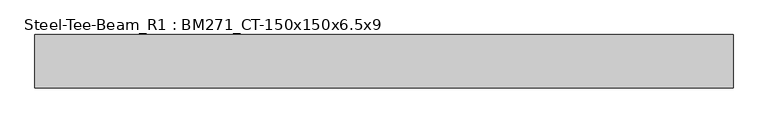
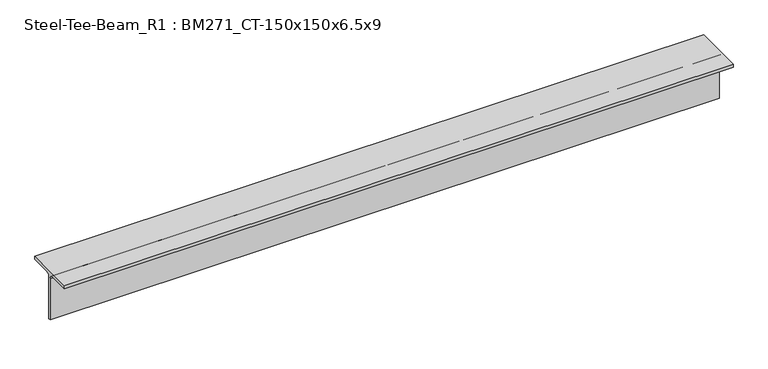
"""IFC4 building model written with IfcOpenShell, lengths in millimetres: member geometry, Steel-Tee-Beam_R1 : BM271_CT-150x150x6.5x9."""

from ifc_helpers import new_model, si_unit, point, frame, frame_2d, origin, place, context, project, spatial, polyline, circle_curve, trimmed, segment, composite_curve, outline, extrude, source, transform, mapped, element, save


def steel_tee_beam_r1_bm271_ct_150x150x6_5x9_9fd703a0(model_context):
    return source(origin(), model_context, "Body", "SweptSolid", [
        extrude(outline(composite_curve([segment(polyline([(75.0, 75.0), (75.0, 66.0), (16.25, 66.0)]), True, "CONTINUOUS"), segment(trimmed(circle_curve(frame_2d((16.25, 53.0)), 13.0), [point((16.25, 66.0))], [point((3.25, 53.0))], True, "CARTESIAN"), True, "CONTINUOUS"), segment(polyline([(3.25, 53.0), (3.25, -75.0), (-3.25, -75.0), (-3.25, 53.0)]), True, "CONTINUOUS"), segment(trimmed(circle_curve(frame_2d((-16.25, 53.0)), 13.0), [point((-3.25, 53.0))], [point((-16.25, 66.0))], True, "CARTESIAN"), True, "CONTINUOUS"), segment(polyline([(-16.25, 66.0), (-75.0, 66.0), (-75.0, 75.0), (75.0, 75.0)]), True, "CONTINUOUS")], self_intersect=False)), frame((-1124.1990532, 0.0, 0.0), z_axis=(1.0, 0.0, 0.0), x_axis=(0.0, 1.0, 0.0)), (0.0, 0.0, 1.0), 1966.5219512),
    ])


if __name__ == "__main__":
    model = new_model("IFC4")
    model_context = context("Model", 3, world=origin())
    ifc_project = project(units=[si_unit("LENGTHUNIT", "METRE", prefix="MILLI")], contexts=[model_context])
    site = spatial("IfcSite", under=ifc_project)
    building = spatial("IfcBuilding", under=site)
    placement = place(None, origin())
    steel_tee_beam_r1_bm271_ct_150x150x6_5x9_shape = steel_tee_beam_r1_bm271_ct_150x150x6_5x9_9fd703a0(model_context)
    element("IfcMember", 1, ObjectType="Steel-Tee-Beam_R1 : BM271_CT-150x150x6.5x9", at=placement, inside=building, context=model_context, shape_type="MappedRepresentation", body=[
        mapped(steel_tee_beam_r1_bm271_ct_150x150x6_5x9_shape, transform((0.0, 0.0, 0.0), x_axis=(1.0, 0.0, 0.0), y_axis=(0.0, 1.0, 0.0), z_axis=(0.0, 0.0, 1.0))),
    ])
    save(model, "model.ifc")

# Revit data of these elements
# Type "Steel-Tee-Beam_R1 : BM271_CT-150x150x6.5x9"
#   Keynote = "CT-150x150x6.5x9"
#   Surface Area = 0.588841 m²/m
#   Section Area = 23.3904 cm²
#   Mass per Unit Length = 18.3614 kg/m
#   Length [instance default] = 1.5240 m
#   bf = 0.1500 m
#   d = 0.1500 m
#   k = 0.0220 m
#   r = 0.0130 m
#   tf = 0.0090 m
#   tw = 0.0065 m
#   hec_material4 [instance default] = none
#   hec_material3 [instance default] = none
#   hec_material2 [instance default] = none
#   hec_material1 [instance default] = none
#   Structural Material [instance default] = Steel, 45-345
#   Assembly Code = ""
# Element 1 (IfcMember, "Steel-Tee-Beam_R1 : BM271_CT-150x150x6.5x9")
#   Structural Material = none
# Materials
#   "Steel, 45-345": class "Metal", colour RGB 189 187 185, transparency 0, Description = "Steel 345 MPa", Cost = 0
